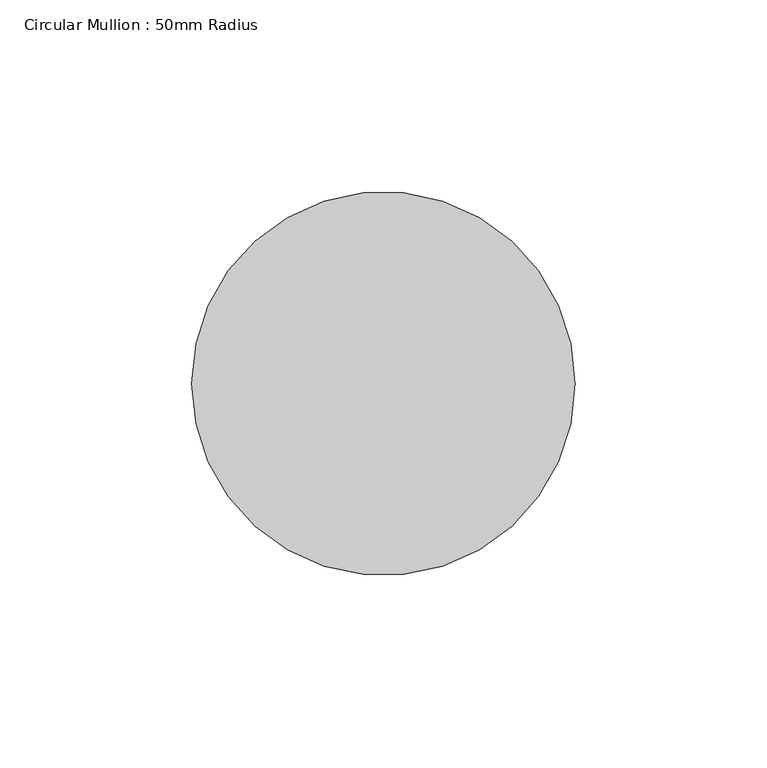
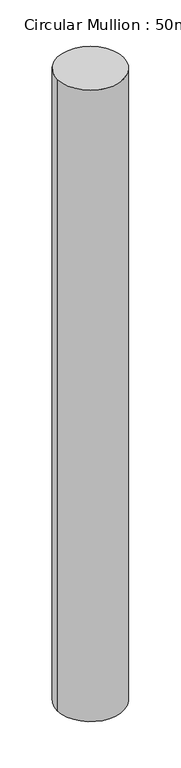
"""IFC4 building model written with IfcOpenShell, lengths in millimetres: member geometry, Circular Mullion : 50mm Radius."""

from ifc_helpers import new_model, si_unit, point, frame, origin, origin_2d, place, context, project, spatial, circle_curve, trimmed, segment, composite_curve, outline, extrude, source, transform, mapped, element, save


def circular_mullion_50mm_radius_805ec990(model_context):
    return source(origin(), model_context, "Body", "SweptSolid", [
        extrude(outline(composite_curve([segment(trimmed(circle_curve(origin_2d(), 50.0), [point((50.0, 0.0))], [point((-50.0, 0.0))], False, "CARTESIAN"), True, "CONTINUOUS"), segment(trimmed(circle_curve(origin_2d(), 50.0), [point((-50.0, 0.0))], [point((50.0, 0.0))], False, "CARTESIAN"), True, "CONTINUOUS")], self_intersect=False)), frame((0.0, 0.0, -1006.8691942), z_axis=(0.0, 0.0, 1.0), x_axis=(1.0, 0.0, 0.0)), (0.0, 0.0, 1.0), 1006.8691942),
    ])


if __name__ == "__main__":
    model = new_model("IFC4")
    model_context = context("Model", 3, world=origin())
    ifc_project = project(units=[si_unit("LENGTHUNIT", "METRE", prefix="MILLI")], contexts=[model_context])
    site = spatial("IfcSite", under=ifc_project)
    building = spatial("IfcBuilding", under=site)
    placement = place(None, origin())
    circular_mullion_50mm_radius_shape = circular_mullion_50mm_radius_805ec990(model_context)
    element("IfcMember", 1, ObjectType="Circular Mullion : 50mm Radius", at=placement, inside=building, context=model_context, shape_type="MappedRepresentation", body=[
        mapped(circular_mullion_50mm_radius_shape, transform((0.0, 0.0, 0.0), x_axis=(1.0, 0.0, 0.0), y_axis=(0.0, 1.0, 0.0), z_axis=(0.0, 0.0, 1.0))),
    ])
    save(model, "model.ifc")

# Revit data of these elements
# Type "Circular Mullion : 50mm Radius"
#   built-in parameter 1007350 = 0.164042 (stored number, unit not read)
# Element 1 (IfcMember, "Circular Mullion : 50mm Radius")
#   Materials on its faces: "Aluminium"
# Materials
#   "Aluminium": class "Metal", colour RGB 247 247 247, transparency 0, Description = "Aluminium 6061", Cost = 0
